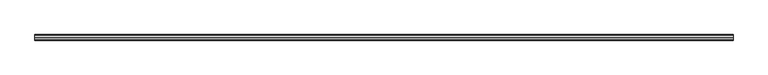
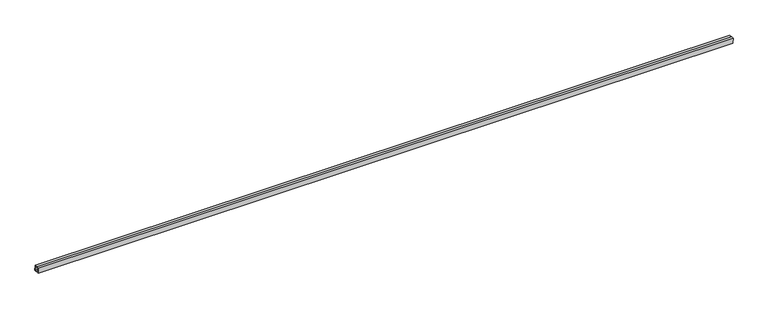
"""IFC4 building model written with IfcOpenShell, lengths in millimetres: proxy geometry, Inner panel:Inner panel:1:Inner panel:1 : Inner panel:Inner panel:300324:2:Inner panel:1:Inner panel:1 : Inner panel:Inner panel:300324:2 : Inner panel:Inner panel:1:Inner panel:1 : Inner panel:Inner panel:300324:300043:13 : Inner panel:Inner panel:1:Inner panel:1 : Inner panel:Inner panel:300324:2:Inner panel:1:Inner panel:1 : Inner panel:Inner panel:300324:2 : Inner panel:Inner panel:1:Inner panel:1 : Inner panel:Inner panel:300324:300043:308120."""

from ifc_helpers import new_model, si_unit, frame, origin, place, context, project, spatial, polyline, outline, extrude, source, transform, mapped, element, save


def generic_models_d36405eb(model_context):
    return source(origin(), model_context, "Body", "SweptSolid", [
        extrude(outline(polyline([(-580608.3153149, 3882.914021), (-580590.0748917, 3883.6740386), (-580588.488768, 3845.6070685), (-580626.5557381, 3844.0209448), (-580628.1418618, 3882.0879149), (-580609.9014386, 3882.8479325), (-580609.8023059, 3880.4687469), (-580625.6635434, 3879.807862), (-580624.2756852, 3846.4992631), (-580590.9670863, 3847.8871214), (-580592.3549446, 3881.1957202), (-580608.2161822, 3880.5348354), (-580608.3153149, 3882.914021)])), frame((588245.3367239, 0.0, 0.0), z_axis=(1.0, 0.0, 0.0), x_axis=(0.0, 1.0, 0.0)), (0.0, 0.0, 1.0), 4876.8),
    ])


if __name__ == "__main__":
    model = new_model("IFC4")
    model_context = context("Model", 3, world=origin())
    ifc_project = project(units=[si_unit("LENGTHUNIT", "METRE", prefix="MILLI")], contexts=[model_context])
    site = spatial("IfcSite", under=ifc_project)
    building = spatial("IfcBuilding", under=site)
    placement = place(None, origin())
    generic_models_shape = generic_models_d36405eb(model_context)
    element("IfcBuildingElementProxy", 1, Name="Inner panel:Inner panel:1:Inner panel:1 : Inner panel:Inner panel:300324:2:Inner panel:1:Inner panel:1 : Inner panel:Inner panel:300324:2 : Inner panel:Inner panel:1:Inner panel:1 : Inner panel:Inner panel:300324:300043:13 : Inner panel:Inner panel:1:Inner panel:1 : Inner panel:Inner panel:300324:2:Inner panel:1:Inner panel:1 : Inner panel:Inner panel:300324:2 : Inner panel:Inner panel:1:Inner panel:1 : Inner panel:Inner panel:300324:300043:308120", ObjectType="Inner panel:Inner panel:1:Inner panel:1 : Inner panel:Inner panel:300324:2:Inner panel:1:Inner panel:1 : Inner panel:Inner panel:300324:2 : Inner panel:Inner panel:1:Inner panel:1 : Inner panel:Inner panel:300324:300043:13 : Inner panel:Inner panel:1:Inner panel:1 : Inner panel:Inner panel:300324:2:Inner panel:1:Inner panel:1 : Inner panel:Inner panel:300324:2 : Inner panel:Inner panel:1:Inner panel:1 : Inner panel:Inner panel:300324:300043:308120", at=placement, inside=building, context=model_context, shape_type="MappedRepresentation", body=[
        mapped(generic_models_shape, transform((0.0, 0.0, 0.0), x_axis=(1.0, 0.0, 0.0), y_axis=(0.0, 1.0, 0.0), z_axis=(0.0, 0.0, 1.0))),
    ])
    save(model, "model.ifc")

# Revit data of these elements
# Type "Inner panel:Inner panel:1:Inner panel:1 : Inner panel:Inner panel:300324:2:Inner panel:1:Inner panel:1 : Inner panel:Inner panel:300324:2 : Inner panel:Inner panel:1:Inner panel:1 : Inner panel:Inner panel:300324:300043:13 : Inner panel:Inner panel:1:Inner panel:1 : Inner panel:Inner panel:300324:2:Inner panel:1:Inner panel:1 : Inner panel:Inner panel:300324:2 : Inner panel:Inner panel:1:Inner panel:1 : Inner panel:Inner panel:300324:300043:308120"
#   NameOverride = "Inner panel:Inner panel:1:Inner panel:1 : Inner panel:Inner panel:300324:2:Inner panel:1:Inner panel:1 : Inner panel:Inner panel:300324:2 : Inner panel:Inner panel:1:Inner panel:1 : Inner panel:Inner panel:300324:300043:308120"
#   ObjectTypeOverride = "Inner panel:1:Inner panel:1 : Inner panel:Inner panel:300324:2 : Inner panel:Inner panel:1:Inner panel:1 : Inner panel:Inner panel:300324:300043"
#   Reference = "Inner panel"
#   Tag = "308120"
# Element 1 (IfcBuildingElementProxy, "Inner panel:Inner panel:1:Inner panel:1 : Inner panel:Inner panel:300324:2:Inner panel:1:Inner panel:1 : Inner panel:Inner panel:300324:2 : Inner panel:Inner panel:1:Inner panel:1 : Inner panel:Inner panel:300324:300043:13 : Inner panel:Inner panel:1:Inner panel:1 : Inner panel:Inner panel:300324:2:Inner panel:1:Inner panel:1 : Inner panel:Inner panel:300324:2 : Inner panel:Inner panel:1:Inner panel:1 : Inner panel:Inner panel:300324:300043:308120")
#   Materials on its faces: "1 1/2\" X 1 1/2\" SPLIT-SEAM SQUARE TUBING (~24\" CANTILEVER FROM C.L. OF GLULAM)"
# Materials
#   "1 1/2\" X 1 1/2\" SPLIT-SEAM SQUARE TUBING (~24\" CANTILEVER FROM C.L. OF GLULAM)": class "Unassigned", colour RGB 202 201 200, transparency 0, Cost = 0
